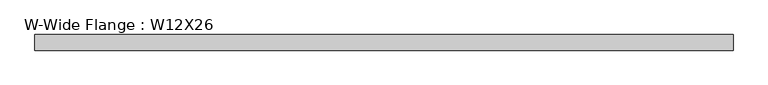
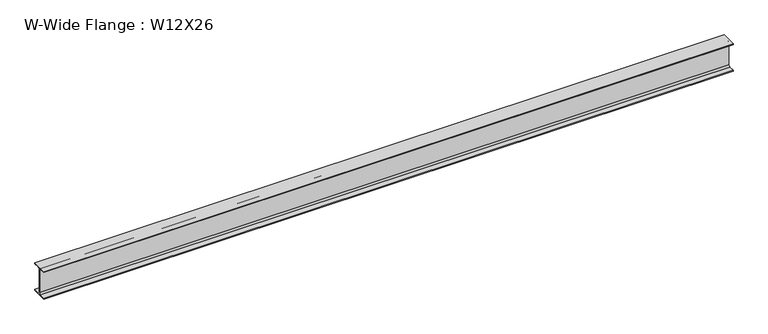
"""IFC4 building model written with IfcOpenShell, lengths in millimetres: beam geometry, W-Wide Flange : W12X26."""

from ifc_helpers import new_model, si_unit, point, frame, frame_2d, origin, place, context, project, spatial, polyline, circle_curve, trimmed, segment, composite_curve, outline, extrude, source, transform, mapped, element, save


def w_wide_flange_w12x26_9f082b63(model_context):
    return source(origin(), model_context, "Body", "SweptSolid", [
        extrude(outline(composite_curve([segment(polyline([(82.4011719, -145.5539063), (82.4011719, -155.178125), (-82.4011719, -155.178125), (-82.4011719, -145.5539063), (-20.2902344, -145.5539063)]), True, "CONTINUOUS"), segment(trimmed(circle_curve(frame_2d((-20.2902344, -128.190625)), 17.3632812), [point((-20.2902344, -145.5539063))], [point((-2.9269531, -128.190625))], True, "CARTESIAN"), True, "CONTINUOUS"), segment(polyline([(-2.9269531, -128.190625), (-2.9269531, 128.190625)]), True, "CONTINUOUS"), segment(trimmed(circle_curve(frame_2d((-20.2902344, 128.190625)), 17.3632812), [point((-2.9269531, 128.190625))], [point((-20.2902344, 145.5539062))], True, "CARTESIAN"), True, "CONTINUOUS"), segment(polyline([(-20.2902344, 145.5539062), (-82.4011719, 145.5539062), (-82.4011719, 155.178125), (82.4011719, 155.178125), (82.4011719, 145.5539062), (20.2902344, 145.5539062)]), True, "CONTINUOUS"), segment(trimmed(circle_curve(frame_2d((20.2902344, 128.190625)), 17.3632812), [point((20.2902344, 145.5539062))], [point((2.9269531, 128.190625))], True, "CARTESIAN"), True, "CONTINUOUS"), segment(polyline([(2.9269531, 128.190625), (2.9269531, -128.190625)]), True, "CONTINUOUS"), segment(trimmed(circle_curve(frame_2d((20.2902344, -128.190625)), 17.3632812), [point((2.9269531, -128.190625))], [point((20.2902344, -145.5539063))], True, "CARTESIAN"), True, "CONTINUOUS"), segment(polyline([(20.2902344, -145.5539063), (82.4011719, -145.5539063)]), True, "CONTINUOUS")], self_intersect=False)), frame((-3590.753424, 0.0, 0.0), z_axis=(1.0, 0.0, 0.0), x_axis=(0.0, 1.0, 0.0)), (0.0, 0.0, 1.0), 7361.8172688),
    ])


if __name__ == "__main__":
    model = new_model("IFC4")
    model_context = context("Model", 3, world=origin())
    ifc_project = project(units=[si_unit("LENGTHUNIT", "METRE", prefix="MILLI")], contexts=[model_context])
    site = spatial("IfcSite", under=ifc_project)
    building = spatial("IfcBuilding", under=site)
    placement = place(None, origin())
    w_wide_flange_w12x26_shape = w_wide_flange_w12x26_9f082b63(model_context)
    element("IfcBeam", 1, ObjectType="W-Wide Flange : W12X26", at=placement, inside=building, context=model_context, shape_type="MappedRepresentation", body=[
        mapped(w_wide_flange_w12x26_shape, transform((0.0, 0.0, 0.0), x_axis=(1.0, 0.0, 0.0), y_axis=(0.0, 1.0, 0.0), z_axis=(0.0, 0.0, 1.0))),
    ])
    save(model, "model.ifc")

# Revit data of these elements
# Type "W-Wide Flange : W12X26"
#   Assembly Code = "B10"
#   W = 26
#   Length [instance default] = 5' - 0"
#   bf = 0' - 6 125/256"
#   d = 1' - 0 7/32"
#   k = 0' - 1 1/16"
#   k2 = 0' - 0 175/256"
#   tf = 0' - 0 97/256"
#   tw = 0' - 0 59/256"
#   A = 0.053125 SF
#   Structural Material [instance default] = none
